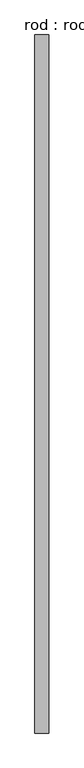
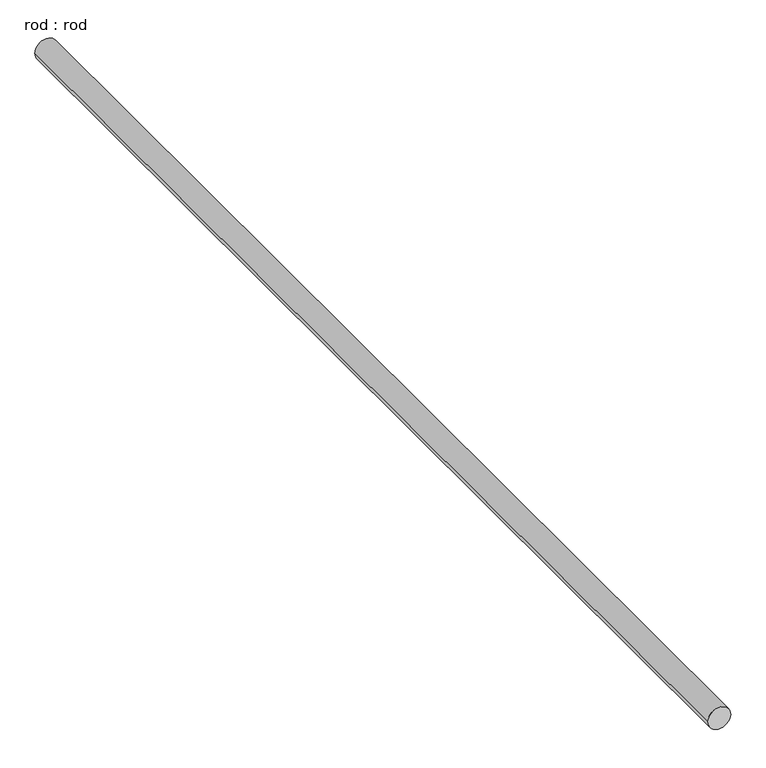
"""IFC4 building model written with IfcOpenShell, lengths in millimetres: proxy geometry, rod : rod."""

from ifc_helpers import new_model, si_unit, point, frame, frame_2d, origin, place, context, project, spatial, circle_curve, trimmed, segment, composite_curve, outline, extrude, source, transform, mapped, element, save


def rod_rod_52191939(model_context):
    return source(origin(), model_context, "Body", "SweptSolid", [
        extrude(outline(composite_curve([segment(trimmed(circle_curve(frame_2d((0.0108462, 0.0)), 200.0), [point((0.0108462, 200.0))], [point((0.0108462, -200.0))], False, "CARTESIAN"), True, "CONTINUOUS"), segment(trimmed(circle_curve(frame_2d((0.0108462, 0.0)), 200.0), [point((0.0108462, -200.0))], [point((0.0108462, 200.0))], False, "CARTESIAN"), True, "CONTINUOUS")], self_intersect=False)), frame((0.0, -6101.7158291, 0.0), z_axis=(0.0, 1.0, 0.0), x_axis=(0.0, 0.0, 1.0)), (0.0, 0.0, 1.0), 20388.8888889),
    ])


if __name__ == "__main__":
    model = new_model("IFC4")
    model_context = context("Model", 3, world=origin())
    ifc_project = project(units=[si_unit("LENGTHUNIT", "METRE", prefix="MILLI")], contexts=[model_context])
    site = spatial("IfcSite", under=ifc_project)
    building = spatial("IfcBuilding", under=site)
    placement = place(None, origin())
    rod_rod_shape = rod_rod_52191939(model_context)
    element("IfcBuildingElementProxy", 1, Name="rod : rod", ObjectType="rod : rod", at=placement, inside=building, context=model_context, shape_type="MappedRepresentation", body=[
        mapped(rod_rod_shape, transform((0.0, 0.0, 0.0), x_axis=(1.0, 0.0, 0.0), y_axis=(0.0, 1.0, 0.0), z_axis=(0.0, 0.0, 1.0))),
    ])
    save(model, "model.ifc")

# Revit data of these elements
# Type "rod : rod"
#   Default Elevation = 0
